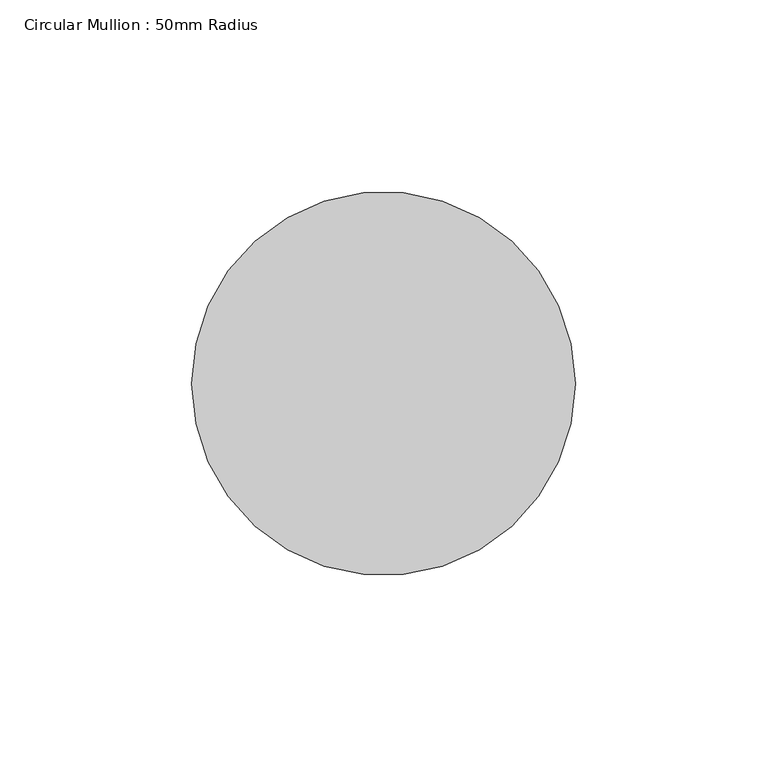
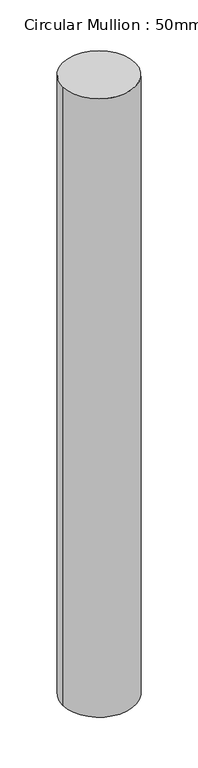
"""IFC4 building model written with IfcOpenShell, lengths in millimetres: member geometry, Circular Mullion : 50mm Radius."""

from ifc_helpers import new_model, si_unit, point, frame, origin, origin_2d, place, context, project, spatial, circle_curve, trimmed, segment, composite_curve, outline, extrude, source, transform, mapped, element, save


def circular_mullion_50mm_radius_f180bd48(model_context):
    return source(origin(), model_context, "Body", "SweptSolid", [
        extrude(outline(composite_curve([segment(trimmed(circle_curve(origin_2d(), 50.0), [point((50.0, 0.0))], [point((-50.0, 0.0))], False, "CARTESIAN"), True, "CONTINUOUS"), segment(trimmed(circle_curve(origin_2d(), 50.0), [point((-50.0, 0.0))], [point((50.0, 0.0))], False, "CARTESIAN"), True, "CONTINUOUS")], self_intersect=False)), frame((0.0, 0.0, -900.4443847), z_axis=(0.0, 0.0, 1.0), x_axis=(1.0, 0.0, 0.0)), (0.0, 0.0, 1.0), 900.4443847),
    ])


if __name__ == "__main__":
    model = new_model("IFC4")
    model_context = context("Model", 3, world=origin())
    ifc_project = project(units=[si_unit("LENGTHUNIT", "METRE", prefix="MILLI")], contexts=[model_context])
    site = spatial("IfcSite", under=ifc_project)
    building = spatial("IfcBuilding", under=site)
    placement = place(None, origin())
    circular_mullion_50mm_radius_shape = circular_mullion_50mm_radius_f180bd48(model_context)
    element("IfcMember", 1, ObjectType="Circular Mullion : 50mm Radius", at=placement, inside=building, context=model_context, shape_type="MappedRepresentation", body=[
        mapped(circular_mullion_50mm_radius_shape, transform((0.0, 0.0, 0.0), x_axis=(1.0, 0.0, 0.0), y_axis=(0.0, 1.0, 0.0), z_axis=(0.0, 0.0, 1.0))),
    ])
    save(model, "model.ifc")

# Revit data of these elements
# Type "Circular Mullion : 50mm Radius"
#   built-in parameter 1007350 = 0.164042 (stored number, unit not read)
# Element 1 (IfcMember, "Circular Mullion : 50mm Radius")
#   Materials on its faces: "Aluminium"
# Materials
#   "Aluminium": class "Metal", colour RGB 247 247 247, transparency 0, Description = "Aluminium 6061", Cost = 0
